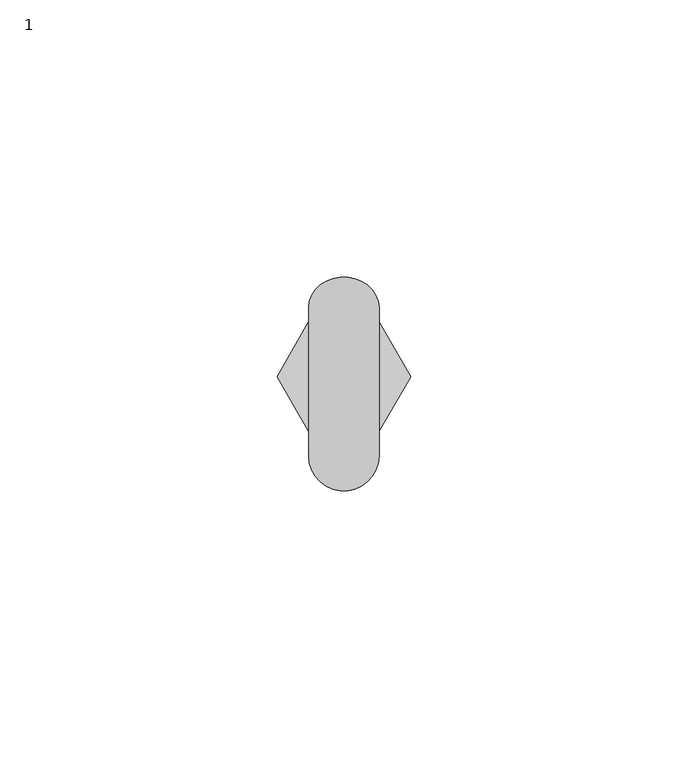
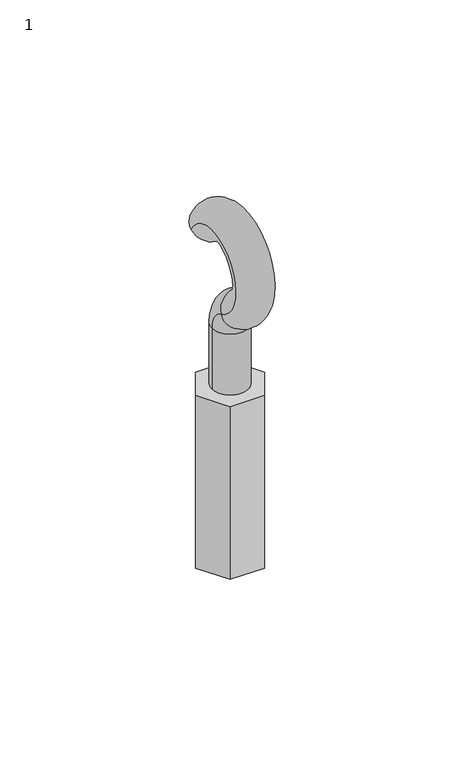
"""IFC4 building model written with IfcOpenShell, lengths in millimetres: proxy geometry, Hanger_Rod-Anvil_International-Weldless_Eye-Fig_248_248L : 1."""

import ifcopenshell
import ifcopenshell.guid

model = None  # the IFC model being written
_history = None  # IfcOwnerHistory: only IFC2X3 demands one
_inside = {}  # id of a spatial element -> (the spatial element, [elements in it])
_under = {}  # id of a project, library or spatial element -> (it, [spatial elements below it])
_declared = {}  # id of a project -> (the project, [libraries it declares])
_typed = {}  # id of a type object -> (the type object, [elements of that type])
_made_of = {}  # id of a material, layer set ... -> (it, [elements and type objects made of it])


def new_model(schema):
    """Start an empty IFC model of exactly this schema.

    Asked for "IFC4X3", IfcOpenShell would pick the latest addendum, in which some entities
    have other attributes; the version numbers below select the first issue.
    IFC2X3 requires an IfcOwnerHistory on every rooted entity: one is made here for all.
    """
    global model, _history
    if schema == "IFC4X3":
        model = ifcopenshell.file(schema_version=(4, 3, 0, 0))
    else:
        model = ifcopenshell.file(schema=schema)
    _inside.clear()
    _under.clear()
    _declared.clear()
    _typed.clear()
    _made_of.clear()
    _history = None
    if model.schema == "IFC2X3":
        org = make("IfcOrganization", Name="unknown")
        user = make(
            "IfcPersonAndOrganization",
            ThePerson=make("IfcPerson", FamilyName="unknown"),
            TheOrganization=org,
        )
        app = make(
            "IfcApplication",
            ApplicationDeveloper=org,
            Version="unknown",
            ApplicationFullName="unknown",
            ApplicationIdentifier="unknown",
        )
        _history = make(
            "IfcOwnerHistory",
            OwningUser=user,
            OwningApplication=app,
            ChangeAction="ADDED",
            CreationDate=0,
        )
    return model


def make(cls, **values):
    """One entity of the class cls with the attributes given. An attribute that is None is left unset."""
    return model.create_entity(
        cls, **{name: value for name, value in values.items() if value is not None}
    )


def rooted(cls, **values):
    """An entity with a GlobalId (a new one), such as an element, a storey or a relation."""
    return make(cls, GlobalId=ifcopenshell.guid.new(), OwnerHistory=_history, **values)


def si_unit(unit_type, name, prefix=None):
    """IfcSIUnit, for example si_unit("LENGTHUNIT", "METRE", prefix="MILLI")."""
    return make("IfcSIUnit", UnitType=unit_type, Prefix=prefix, Name=name)


def assignment(units):
    """IfcUnitAssignment: the units of a project."""
    return None if units is None else make("IfcUnitAssignment", Units=units)


def point(xyz):
    """IfcCartesianPoint."""
    return None if xyz is None else make("IfcCartesianPoint", Coordinates=xyz)


def direction(xyz):
    """IfcDirection."""
    return None if xyz is None else make("IfcDirection", DirectionRatios=xyz)


def frame(location, z_axis=None, x_axis=None):
    """IfcAxis2Placement3D, a coordinate frame: its origin and axes. An axis left out is left unset."""
    return make(
        "IfcAxis2Placement3D",
        Location=point(location),
        Axis=direction(z_axis),
        RefDirection=direction(x_axis),
    )


def origin():
    """The frame at (0, 0, 0) with its axes left unset."""
    return frame((0.0, 0.0, 0.0))


def origin_with_axes():
    """The frame at (0, 0, 0) with the z axis (0, 0, 1) and the x axis (1, 0, 0) written out."""
    return frame((0.0, 0.0, 0.0), z_axis=(0.0, 0.0, 1.0), x_axis=(1.0, 0.0, 0.0))


def place(relative_to, where):
    """IfcLocalPlacement: puts the frame where relative to a parent placement (None: the world)."""
    return make(
        "IfcLocalPlacement", PlacementRelTo=relative_to, RelativePlacement=where
    )


def context(
    kind, dimensions, precision=None, world=None, true_north=None, identifier=None
):
    """IfcGeometricRepresentationContext, for example the 3D "Model" context."""
    return make(
        "IfcGeometricRepresentationContext",
        ContextIdentifier=identifier,
        ContextType=kind,
        CoordinateSpaceDimension=dimensions,
        Precision=precision,
        WorldCoordinateSystem=world,
        TrueNorth=true_north,
    )


def project(units=None, contexts=None):
    """IfcProject with its units and contexts."""
    return rooted(
        "IfcProject",
        Name="project",
        RepresentationContexts=contexts,
        UnitsInContext=assignment(units),
    )


def spatial(cls, under=None, at=None, **own):
    """A site, building, storey or space (cls), placed at a placement, below another one or the project."""
    s = rooted(cls, ObjectPlacement=at, **own)
    if under is not None:
        _under.setdefault(under.id(), (under, []))[1].append(s)
    return s


def polyline(points):
    """IfcPolyline through the points."""
    return make("IfcPolyline", Points=[point(p) for p in points])


def circle_curve(where, radius):
    """IfcCircle in the frame where."""
    return make("IfcCircle", Position=where, Radius=radius)


def ellipse_curve(where, semi_axis1, semi_axis2):
    """IfcEllipse in the frame where."""
    return make(
        "IfcEllipse", Position=where, SemiAxis1=semi_axis1, SemiAxis2=semi_axis2
    )


def trimmed(basis, trim1, trim2, sense, master):
    """IfcTrimmedCurve: the piece of a basis curve between two trims."""
    return make(
        "IfcTrimmedCurve",
        BasisCurve=basis,
        Trim1=trim1,
        Trim2=trim2,
        SenseAgreement=sense,
        MasterRepresentation=master,
    )


def outline(outer, holes=None, kind="AREA"):
    """IfcArbitraryClosedProfileDef: a profile drawn as a closed curve; with holes, ...WithVoids."""
    if holes is None:
        return make("IfcArbitraryClosedProfileDef", ProfileType=kind, OuterCurve=outer)
    return make(
        "IfcArbitraryProfileDefWithVoids",
        ProfileType=kind,
        OuterCurve=outer,
        InnerCurves=holes,
    )


def extrude(swept, where, along, depth):
    """IfcExtrudedAreaSolid: the profile swept, set in the frame where, extruded along a direction by depth."""
    return make(
        "IfcExtrudedAreaSolid",
        SweptArea=swept,
        Position=where,
        ExtrudedDirection=direction(along),
        Depth=depth,
    )


def shape(context_of_items, identifier, shape_type, items):
    """IfcShapeRepresentation: the items that make up one representation, for example the "Body"."""
    return make(
        "IfcShapeRepresentation",
        ContextOfItems=context_of_items,
        RepresentationIdentifier=identifier,
        RepresentationType=shape_type,
        Items=items,
    )


def source(mapping_origin, context_of_items, identifier, shape_type, items):
    """IfcRepresentationMap: a shape defined once, which mapped items show again and again."""
    return make(
        "IfcRepresentationMap",
        MappingOrigin=mapping_origin,
        MappedRepresentation=shape(context_of_items, identifier, shape_type, items),
    )


def transform(
    local_origin,
    x_axis=None,
    y_axis=None,
    z_axis=None,
    scale=None,
    scale2=None,
    scale3=None,
    uniform=True,
):
    """IfcCartesianTransformationOperator3D, or its non-uniform kind. x_axis, y_axis, z_axis: its Axis1, 2, 3."""
    if uniform:
        return make(
            "IfcCartesianTransformationOperator3D",
            Axis1=direction(x_axis),
            Axis2=direction(y_axis),
            LocalOrigin=point(local_origin),
            Scale=scale,
            Axis3=direction(z_axis),
        )
    return make(
        "IfcCartesianTransformationOperator3DnonUniform",
        Axis1=direction(x_axis),
        Axis2=direction(y_axis),
        LocalOrigin=point(local_origin),
        Scale=scale,
        Axis3=direction(z_axis),
        Scale2=scale2,
        Scale3=scale3,
    )


def mapped(mapping_source, mapping_target):
    """IfcMappedItem: shows the shape of a source again, moved by a transform."""
    return make(
        "IfcMappedItem", MappingSource=mapping_source, MappingTarget=mapping_target
    )


def made_of(thing, what):
    """Note that an element or type object is made of a material, layer set ...; save() writes the relation."""
    if what is not None:
        _made_of.setdefault(what.id(), (what, []))[1].append(thing)
    return thing


def element(
    cls,
    number,
    at=None,
    inside=None,
    cuts=None,
    type_object=None,
    material=None,
    context=None,
    identifier="Body",
    shape_type=None,
    held_by="IfcProductDefinitionShape",
    body=None,
    shapes=None,
    **own,
):
    """One element of the class cls, such as IfcWall. Its Tag is "e" and its number.

    at: its placement. inside: the storey or other place that contains it. cuts: it is an
    opening in that element (IfcRelVoidsElement). A single representation is given by context,
    identifier, shape_type and body (its items); several are given by shapes. held_by: the class
    of the entity that holds the representations. save() writes the other relations.
    """
    e = rooted(cls, Tag="e%d" % number, ObjectPlacement=at, **own)
    if body is not None:
        shapes = [shape(context, identifier, shape_type, body)]
    if shapes is not None:
        e.Representation = make(held_by, Representations=shapes)
    if inside is not None:
        _inside.setdefault(inside.id(), (inside, []))[1].append(e)
    if cuts is not None:
        rooted(
            "IfcRelVoidsElement", RelatingBuildingElement=cuts, RelatedOpeningElement=e
        )
    if type_object is not None:
        _typed.setdefault(type_object.id(), (type_object, []))[1].append(e)
    return made_of(e, material)


def aggregate(whole, parts):
    """IfcRelAggregates: a whole, such as a stair, and the parts it consists of."""
    return rooted("IfcRelAggregates", RelatingObject=whole, RelatedObjects=parts)


def save(model, path):
    """Write the relations noted so far, then the file.

    IfcRelAggregates (storeys below a building ...), IfcRelContainedInSpatialStructure (elements
    in a storey), IfcRelDefinesByType, IfcRelAssociatesMaterial and IfcRelDeclares: one each for
    every whole, place, type object, material and project.
    """
    for whole, parts in _under.values():
        aggregate(whole, parts)
    for where, things in _inside.values():
        rooted(
            "IfcRelContainedInSpatialStructure",
            RelatedElements=things,
            RelatingStructure=where,
        )
    for kind, things in _typed.values():
        rooted("IfcRelDefinesByType", RelatedObjects=things, RelatingType=kind)
    for what, things in _made_of.values():
        rooted("IfcRelAssociatesMaterial", RelatedObjects=things, RelatingMaterial=what)
    for by, libraries in _declared.values():
        rooted("IfcRelDeclares", RelatingContext=by, RelatedDefinitions=libraries)
    model.write(path)


def plane_surface(at):
    """IfcPlane: the flat surface through the origin of the frame at, square to its z axis."""
    return make("IfcPlane", Position=at)


def cylinder_surface(at, radius):
    """IfcCylindricalSurface: all points at the distance radius from the z axis of the frame at."""
    return make("IfcCylindricalSurface", Position=at, Radius=radius)


def revolved_surface(curve, axis_point, axis_direction):
    """IfcSurfaceOfRevolution: the curve turned about the line through axis_point along axis_direction."""
    return make(
        "IfcSurfaceOfRevolution",
        SweptCurve=make("IfcArbitraryOpenProfileDef", ProfileType="CURVE", Curve=curve),
        AxisPosition=make("IfcAxis1Placement", Location=point(axis_point), Axis=direction(axis_direction)),
    )


def advanced_brep(points, edges, surfaces, faces):
    """IfcAdvancedBrep: a solid bounded by faces that lie on surfaces and meet in shared edges.

    An edge is (start, end): straight between two places in points (the first is 0);
    or (start, end, curve); or (start, end, curve, False) where it runs against its curve.
    A face is (place in surfaces, loops), or (place, loops, False) where it looks against
    its surface's normal. A loop lists edges by number (the first is 1), with a minus sign
    where the edge is run from its end to its start. The first loop is the outer one.
    """
    corners = [point(p) for p in points]
    vertices = [make("IfcVertexPoint", VertexGeometry=c) for c in corners]
    made = []
    for start, end, *more in edges:
        made.append(
            make(
                "IfcEdgeCurve",
                EdgeStart=vertices[start],
                EdgeEnd=vertices[end],
                EdgeGeometry=more[0] if more else make("IfcPolyline", Points=[corners[start], corners[end]]),
                SameSense=more[1] if len(more) > 1 else True,
            )
        )
    hull = []
    for where, loops, *sense in faces:
        bounds = []
        for j, loop in enumerate(loops):
            ring = [make("IfcOrientedEdge", EdgeElement=made[abs(k) - 1], Orientation=k > 0) for k in loop]
            bounds.append(
                make(
                    "IfcFaceOuterBound" if j == 0 else "IfcFaceBound",
                    Bound=make("IfcEdgeLoop", EdgeList=ring),
                    Orientation=True,
                )
            )
        hull.append(make("IfcAdvancedFace", Bounds=bounds, FaceSurface=surfaces[where], SameSense=sense[0] if sense else True))
    return make("IfcAdvancedBrep", Outer=make("IfcClosedShell", CfsFaces=hull))


def proxy_1_632f9fa5(model_context):
    return source(origin(), model_context, "Body", "SolidModel", [
        extrude(outline(polyline([(-12.0281557, 0.0), (-6.0140778, 10.4166884), (6.0140778, 10.4166884), (12.0281557, 0.0), (6.0140778, -10.4166884), (-6.0140778, -10.4166884), (-12.0281557, 0.0)])), origin_with_axes(), (0.0, 0.0, 1.0), 63.5),
        advanced_brep(
        [(-6.35, 0.0, 63.5), (6.35, 0.0, 63.5), (6.35, 0.0, 86.1254833), (-6.35, 0.0, 86.1254833), (-6.35, 12.4384419, 114.9797808), (6.35, 12.4384419, 114.9797808), (6.35, -5.715, 94.85529), (-6.35, -5.715, 94.85529)],
        [
            (0, 1, circle_curve(frame((0.0, 0.0, 63.5), z_axis=(0.0, 0.0, -1.0), x_axis=(1.0, 0.0, 0.0)), 6.35)),
            (1, 0, circle_curve(frame((0.0, 0.0, 63.5), z_axis=(0.0, 0.0, -1.0), x_axis=(1.0, 0.0, 0.0)), 6.35)),
            (2, 1),
            (0, 3),
            (3, 2, circle_curve(frame((0.0, 0.0, 86.1254833), z_axis=(0.0, 0.0, -1.0), x_axis=(1.0, 0.0, 0.0)), 6.35)),
            (2, 3, circle_curve(frame((0.0, 0.0, 86.1254833), z_axis=(0.0, 0.0, -1.0), x_axis=(1.0, 0.0, 0.0)), 6.35)),
            (4, 5, circle_curve(frame((0.0, 12.4384419, 114.9797808), z_axis=(0.0, 0.49202315445778766, -0.8705821130010701), x_axis=(1.0, 0.0, 0.0)), 6.35)),
            (5, 4, circle_curve(frame((0.0, 12.4384419, 114.9797808), z_axis=(0.0, 0.49202315445778766, -0.8705821130010701), x_axis=(1.0, 0.0, 0.0)), 6.35)),
            (6, 7, circle_curve(frame((0.0, -5.715, 94.85529), z_axis=(0.0, -0.9165151389911654, 0.4000000000000058), x_axis=(1.0, 0.0, 0.0)), 6.35)),
            (7, 4, circle_curve(frame((-6.35, 0.0, 107.95), z_axis=(-1.0, 0.0, 0.0), x_axis=(0.0, 0.8705821130010701, 0.4920231544577876)), 14.2875)),
            (5, 6, circle_curve(frame((6.35, 0.0, 107.95), z_axis=(1.0, 0.0, 0.0), x_axis=(0.0, 0.8705821130010701, 0.4920231544577876)), 14.2875)),
            (7, 6, circle_curve(frame((0.0, -5.715, 94.85529), z_axis=(0.0, -0.9165151389911654, 0.4000000000000058), x_axis=(1.0, 0.0, 0.0)), 6.35)),
            (3, 7, circle_curve(frame((-6.35, -9.525, 86.1254833), z_axis=(1.0, 0.0, 0.0), x_axis=(0.0, 0.4000000000000002, 0.9165151389911679)), 9.525)),
            (6, 2, circle_curve(frame((6.35, -9.525, 86.1254833), z_axis=(-1.0, 0.0, 0.0), x_axis=(0.0, 0.4000000000000002, 0.9165151389911679)), 9.525)),
        ],
        [
            plane_surface(frame((0.0, 6.35, 63.5), z_axis=(0.0, 0.0, -1.0), x_axis=(1.0, 0.0, 0.0))),
            cylinder_surface(frame((0.0, 0.0, 86.1254833), z_axis=(0.0, 0.0, 1.0), x_axis=(1.0, 0.0, 0.0)), 6.35),
            plane_surface(frame((0.0, 6.9102455, 111.8554338), z_axis=(0.0, 0.49202315445778766, -0.8705821130010701), x_axis=(1.0, 0.0, 0.0))),
            revolved_surface(trimmed(ellipse_curve(frame((0.0, 12.4384419, 114.9797808), z_axis=(0.0, -0.49202315445778766, 0.8705821130010701), x_axis=(1.0, 0.0, 0.0)), 6.35, 6.35), [point((-6.35, 12.4384419, 114.9797808))], [point((6.35, 12.4384419, 114.9797808))], True, "CARTESIAN"), (0.0, 0.0, 107.95), (-1.0, 0.0, 0.0)),
            revolved_surface(trimmed(ellipse_curve(frame((0.0, 12.4384419, 114.9797808), z_axis=(0.0, -0.49202315445778766, 0.8705821130010701), x_axis=(1.0, 0.0, 0.0)), 6.35, 6.35), [point((6.35, 12.4384419, 114.9797808))], [point((-6.35, 12.4384419, 114.9797808))], True, "CARTESIAN"), (0.0, 0.0, 107.95), (-1.0, 0.0, 0.0)),
            revolved_surface(trimmed(ellipse_curve(frame((0.0, -5.715, 94.85529), z_axis=(0.0, 0.9165151389911679, -0.4000000000000001), x_axis=(1.0, 0.0, 0.0)), 6.35, 6.35), [point((-6.35, -5.715, 94.85529))], [point((6.35, -5.715, 94.85529))], True, "CARTESIAN"), (0.0, -9.525, 86.1254833), (1.0, 0.0, 0.0)),
            revolved_surface(trimmed(ellipse_curve(frame((0.0, -5.715, 94.85529), z_axis=(0.0, 0.9165151389911679, -0.4000000000000001), x_axis=(1.0, 0.0, 0.0)), 6.35, 6.35), [point((6.35, -5.715, 94.85529))], [point((-6.35, -5.715, 94.85529))], True, "CARTESIAN"), (0.0, -9.525, 86.1254833), (1.0, 0.0, 0.0)),
        ],
        [
            (0, [[1, 2]]),
            (1, [[3, -1, 4, 5]]),
            (1, [[-4, -2, -3, 6]]),
            (2, [[7, 8]]),
            (3, [[9, 10, -8, 11]]),
            (4, [[12, -11, -7, -10]]),
            (5, [[-5, 13, -9, 14]]),
            (6, [[-6, -14, -12, -13]]),
        ],
    ),
    ])


if __name__ == "__main__":
    model = new_model("IFC4")
    model_context = context("Model", 3, world=origin())
    ifc_project = project(units=[si_unit("LENGTHUNIT", "METRE", prefix="MILLI")], contexts=[model_context])
    site = spatial("IfcSite", under=ifc_project)
    building = spatial("IfcBuilding", under=site)
    placement = place(None, origin())
    proxy_1_shape = proxy_1_632f9fa5(model_context)
    element("IfcBuildingElementProxy", 1, Name="Hanger_Rod-Anvil_International-Weldless_Eye-Fig_248_248L : 1", ObjectType="Hanger_Rod-Anvil_International-Weldless_Eye-Fig_248_248L : 1", at=placement, inside=building, context=model_context, shape_type="MappedRepresentation", body=[
        mapped(proxy_1_shape, transform((0.0, 0.0, 0.0), x_axis=(1.0, 0.0, 0.0), y_axis=(0.0, 1.0, 0.0), z_axis=(0.0, 0.0, 1.0))),
    ])
    save(model, "model.ifc")

# Revit data of these elements
# Type "Hanger_Rod-Anvil_International-Weldless_Eye-Fig_248_248L : 1"
#   z Error Text [instance default] = "Not Available"
#   URL = "http://www.anvilintl.com/"
#   Product data url = "https://bimobject.com/anvil-international/product/anvil-fig-248"
#   Product Page URL = "http://www.anvilintl.com/products/pipe-hangers-and-hardware/hanger-rods-and-accessories/248-figure-threaded-eye-rod-not-welded---rh"
#   Product Documentation Link = "http://www.anvilintl.com/usercontent/submittal-info-sheet/9579_HG-SUB-FIG248_FIG248L.pdf"
#   Part Number [instance default] = "Contact Anvil Sales for More Options"
#   Part Description [instance default] = "Contact Anvil Sales for More Options"
#   Model Disclaimer = "Contact Anvil International for More Information"
#   Model = "See Part Number"
#   Manufacturer = "Anvil International"
#   Family Version = "1.0"
#   Equipment Number [instance default] = ""
#   Equipment Abbreviation = "HR"
#   Description = "See Part Description"
#   Date Modified = "March 13, 2015"
#   Date Created = "March 13, 2015"
#   Copyright = "Copyright ©2015 Anvil International"
#   z Thread Length [instance default] = 0' - 9"
#   z Overall Width [instance default] = 0' - 2 1/4"
#   z Overall Height [instance default] = 1' - 7"
#   z Overall Depth [instance default] = 0' - 7"
#   z Offset [instance default] = 0' - 0"
#   z Eye to End [instance default] = 1' - 3 1/2"
#   z Eye Radius [instance default] = 0' - 1 1/4"
#   z Eye Diameter [instance default] = 0' - 2 1/2"
#   z Error Box Width [instance default] = 0' - 0.1"
#   z Error Box Height [instance default] = 0' - 0.1"
#   z Error Box Depth [instance default] = 0' - 0.1"
#   z Curve Radius [instance default] = 0' - 2 1/2"
#   z Curve Offset X [instance default] = 0' - 1 3/8"
#   z Curve Offset [instance default] = 0' - 3.48882"
#   z Bolt Radius [instance default] = 0' - 1 1/8"
#   Weight Capacity [instance default] = 10.90 kip
#   Rod Length Actual [instance default] = 0' - 6"
#   Rod Diameter Desired [instance default] = 0' - 2 1/4"
#   Rod Length Desired [instance default] = 0' - 6"
#   Rod Diameter Actual [instance default] = 0' - 2 1/4"
#   Maximum Working Temperature [instance default] = 650 °F
#   Default Elevation = 4' - 0"
#   z Type Thread [instance default] = 1
#   z Type Material = 1
#   z Error [instance default] = no
#   Has Right Hand Threads [instance default] = yes
#   Has Left Hand Threads [instance default] = no
#   Product Material = Carbon Steel - Anvil
# Element 1 (IfcBuildingElementProxy, "Hanger_Rod-Anvil_International-Weldless_Eye-Fig_248_248L : 1")
#   z Error Text = "Error: Size Not Available"
#   Part Number = "Error: Size Not Available"
#   Part Description = "Error: Size Not Available"
#   z Thread Length = 0' - 2 1/2"
#   z Overall Width = 0' - 0 1/2"
#   z Overall Height = 0' - 5 1/16"
#   z Overall Depth = 0' - 1 5/8"
#   z Eye to End = 0' - 4 1/4"
#   z Eye Radius = 0' - 0 5/16"
#   z Eye Diameter = 0' - 0 5/8"
#   z Error Box Width = 0' - 5 1/2"
#   z Error Box Height = 0' - 10 1/16"
#   z Error Box Depth = 0' - 6 5/8"
#   z Curve Radius = 0' - 0 5/8"
#   z Curve Offset X = 0' - 0 3/8"
#   z Curve Offset = 0' - 0.85923"
#   z Bolt Radius = 0' - 0 1/4"
#   Weight Capacity = 0.24 kip
#   Rod Length Actual = 4' - 6"
#   Rod Diameter Desired = 0' - 0 1/2"
#   Rod Length Desired = 4' - 3 1/2"
#   Rod Diameter Actual = 0' - 0 1/2"
#   z Error = yes
#   Materials on its faces: "THREADED HEX COUPLING (RAW STEEL)", "1/2\" STEEL EYE BOLT (RAW STEEL)"
# Materials
#   "Carbon Steel - Anvil": class "Unassigned", colour RGB 189 187 185, transparency 0
#   "THREADED HEX COUPLING (RAW STEEL)": class "Unassigned", colour RGB 189 187 185, transparency 0, Cost = 0
#   "1/2\" STEEL EYE BOLT (RAW STEEL)": class "Unassigned", colour RGB 189 187 185, transparency 0, Cost = 0
